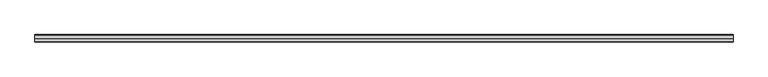
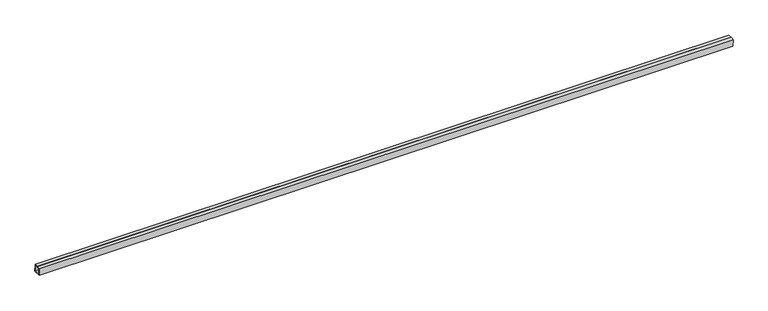
"""IFC4 building model written with IfcOpenShell, lengths in millimetres: proxy geometry, Inner panel:Inner panel:1:Inner panel:1 : Inner panel:Inner panel:300324:2:Inner panel:1:Inner panel:1 : Inner panel:Inner panel:300324:2 : Inner panel:Inner panel:1:Inner panel:1 : Inner panel:Inner panel:300324:300043:24 : Inner panel:Inner panel:1:Inner panel:1 : Inner panel:Inner panel:300324:2:Inner panel:1:Inner panel:1 : Inner panel:Inner panel:300324:2 : Inner panel:Inner panel:1:Inner panel:1 : Inner panel:Inner panel:300324:300043:308120."""

from ifc_helpers import new_model, si_unit, frame, origin, place, context, project, spatial, polyline, outline, extrude, source, transform, mapped, element, save


def generic_models_d45d1c03(model_context):
    return source(origin(), model_context, "Body", "SweptSolid", [
        extrude(outline(polyline([(-565838.6723382, 8901.5279981), (-565820.431915, 8902.2880157), (-565818.8457913, 8864.2210456), (-565856.9127614, 8862.6349219), (-565858.4988851, 8900.701892), (-565840.2584619, 8901.4619096), (-565840.1593292, 8899.082724), (-565856.0205667, 8898.4218391), (-565854.6327085, 8865.1132403), (-565821.3241096, 8866.5010985), (-565822.7119679, 8899.8096974), (-565838.5732055, 8899.1488125), (-565838.6723382, 8901.5279981)])), frame((593141.1867242, 0.0, 0.0), z_axis=(1.0, 0.0, 0.0), x_axis=(0.0, 1.0, 0.0)), (0.0, 0.0, 1.0), 3657.6),
    ])


if __name__ == "__main__":
    model = new_model("IFC4")
    model_context = context("Model", 3, world=origin())
    ifc_project = project(units=[si_unit("LENGTHUNIT", "METRE", prefix="MILLI")], contexts=[model_context])
    site = spatial("IfcSite", under=ifc_project)
    building = spatial("IfcBuilding", under=site)
    placement = place(None, origin())
    generic_models_shape = generic_models_d45d1c03(model_context)
    element("IfcBuildingElementProxy", 1, Name="Inner panel:Inner panel:1:Inner panel:1 : Inner panel:Inner panel:300324:2:Inner panel:1:Inner panel:1 : Inner panel:Inner panel:300324:2 : Inner panel:Inner panel:1:Inner panel:1 : Inner panel:Inner panel:300324:300043:24 : Inner panel:Inner panel:1:Inner panel:1 : Inner panel:Inner panel:300324:2:Inner panel:1:Inner panel:1 : Inner panel:Inner panel:300324:2 : Inner panel:Inner panel:1:Inner panel:1 : Inner panel:Inner panel:300324:300043:308120", ObjectType="Inner panel:Inner panel:1:Inner panel:1 : Inner panel:Inner panel:300324:2:Inner panel:1:Inner panel:1 : Inner panel:Inner panel:300324:2 : Inner panel:Inner panel:1:Inner panel:1 : Inner panel:Inner panel:300324:300043:24 : Inner panel:Inner panel:1:Inner panel:1 : Inner panel:Inner panel:300324:2:Inner panel:1:Inner panel:1 : Inner panel:Inner panel:300324:2 : Inner panel:Inner panel:1:Inner panel:1 : Inner panel:Inner panel:300324:300043:308120", at=placement, inside=building, context=model_context, shape_type="MappedRepresentation", body=[
        mapped(generic_models_shape, transform((0.0, 0.0, 0.0), x_axis=(1.0, 0.0, 0.0), y_axis=(0.0, 1.0, 0.0), z_axis=(0.0, 0.0, 1.0))),
    ])
    save(model, "model.ifc")

# Revit data of these elements
# Type "Inner panel:Inner panel:1:Inner panel:1 : Inner panel:Inner panel:300324:2:Inner panel:1:Inner panel:1 : Inner panel:Inner panel:300324:2 : Inner panel:Inner panel:1:Inner panel:1 : Inner panel:Inner panel:300324:300043:24 : Inner panel:Inner panel:1:Inner panel:1 : Inner panel:Inner panel:300324:2:Inner panel:1:Inner panel:1 : Inner panel:Inner panel:300324:2 : Inner panel:Inner panel:1:Inner panel:1 : Inner panel:Inner panel:300324:300043:308120"
#   NameOverride = "Inner panel:Inner panel:1:Inner panel:1 : Inner panel:Inner panel:300324:2:Inner panel:1:Inner panel:1 : Inner panel:Inner panel:300324:2 : Inner panel:Inner panel:1:Inner panel:1 : Inner panel:Inner panel:300324:300043:308120"
#   ObjectTypeOverride = "Inner panel:1:Inner panel:1 : Inner panel:Inner panel:300324:2 : Inner panel:Inner panel:1:Inner panel:1 : Inner panel:Inner panel:300324:300043"
#   Reference = "Inner panel"
#   Tag = "308120"
# Element 1 (IfcBuildingElementProxy, "Inner panel:Inner panel:1:Inner panel:1 : Inner panel:Inner panel:300324:2:Inner panel:1:Inner panel:1 : Inner panel:Inner panel:300324:2 : Inner panel:Inner panel:1:Inner panel:1 : Inner panel:Inner panel:300324:300043:24 : Inner panel:Inner panel:1:Inner panel:1 : Inner panel:Inner panel:300324:2:Inner panel:1:Inner panel:1 : Inner panel:Inner panel:300324:2 : Inner panel:Inner panel:1:Inner panel:1 : Inner panel:Inner panel:300324:300043:308120")
#   Materials on its faces: "1 1/2\" X 1 1/2\" SPLIT-SEAM SQUARE TUBING (~24\" CANTILEVER FROM C.L. OF GLULAM)"
# Materials
#   "1 1/2\" X 1 1/2\" SPLIT-SEAM SQUARE TUBING (~24\" CANTILEVER FROM C.L. OF GLULAM)": class "Unassigned", colour RGB 202 201 200, transparency 0, Cost = 0
